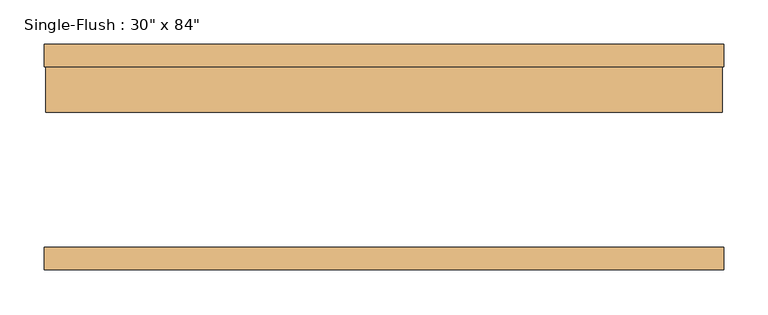
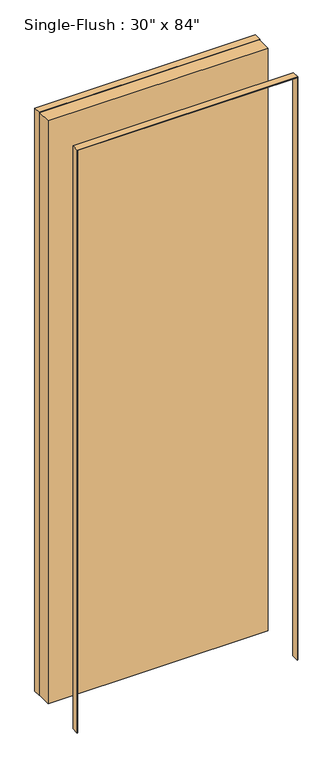
"""IFC4 building model written with IfcOpenShell, lengths in millimetres: door geometry."""

from ifc_helpers import new_model, si_unit, frame, origin, origin_with_axes, place, context, project, spatial, polyline, outline, extrude, source, transform, mapped, element, save


def door_48872733(model_context):
    return source(origin(), model_context, "Body", "SweptSolid", [
        extrude(outline(polyline([(2135.1875, -382.5875), (0.0, -382.5875), (0.0, -381.0), (2133.6, -381.0), (2133.6, 381.0), (0.0, 381.0), (0.0, 382.5875), (2135.1875, 382.5875), (2135.1875, -382.5875)])), frame((0.0, 101.6, 0.0), z_axis=(0.0, 1.0, 0.0), x_axis=(0.0, 0.0, 1.0)), (0.0, 0.0, 1.0), 25.4),
        extrude(outline(polyline([(2135.1875, 382.5875), (2135.1875, -382.5875), (0.0, -382.5875), (0.0, -381.0), (2133.6, -381.0), (2133.6, 381.0), (0.0, 381.0), (0.0, 382.5875), (2135.1875, 382.5875)])), frame((0.0, -127.0, 0.0), z_axis=(0.0, 1.0, 0.0), x_axis=(0.0, 0.0, 1.0)), (0.0, 0.0, 1.0), 25.4),
        extrude(outline(polyline([(381.0, 50.8), (-381.0, 50.8), (-381.0, 101.6), (381.0, 101.6), (381.0, 50.8)])), origin_with_axes(), (0.0, 0.0, 1.0), 2133.6),
    ])


if __name__ == "__main__":
    model = new_model("IFC4")
    model_context = context("Model", 3, world=origin())
    ifc_project = project(units=[si_unit("LENGTHUNIT", "METRE", prefix="MILLI")], contexts=[model_context])
    site = spatial("IfcSite", under=ifc_project)
    building = spatial("IfcBuilding", under=site)
    placement = place(None, origin())
    door_shape = door_48872733(model_context)
    element("IfcDoor", 1, ObjectType="Single-Flush : 30\" x 84\"", at=placement, inside=building, context=model_context, shape_type="MappedRepresentation", body=[
        mapped(door_shape, transform((0.0, 0.0, 0.0), x_axis=(1.0, 0.0, 0.0), y_axis=(0.0, 1.0, 0.0), z_axis=(0.0, 0.0, 1.0))),
    ])
    save(model, "model.ifc")

# Revit data of these elements
# Type "Single-Flush : 30\" x 84\""
#   Type Mark = "4"
#   Assembly Code = "C1020"
#   Thickness = 0' - 2"
#   Height = 7' - 0"
#   Trim Projection Ext = 0' - 1"
#   Trim Projection Int = 0' - 1"
#   Trim Width = 0' - 0 1/16"
#   Width = 2' - 6"
#   Door Material = Door - Panel
#   Frame Material = Door - Frame
#   Function = (empty or 0)
#   Wall Closure = (empty or 0)
# Element 1 (IfcDoor, "Single-Flush : 30\" x 84\"")
#   Materials on its faces: "Door - Frame", "Door - Panel"
# Materials
#   "Door - Panel": class "Wood", colour RGB 210 159 95, transparency 0
#   "Door - Frame": class "Miscellaneous", colour RGB 118 70 51, transparency 0
